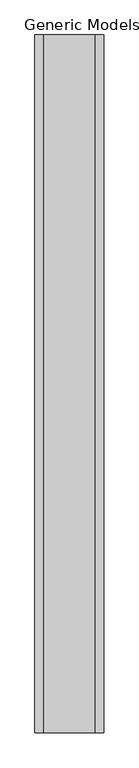
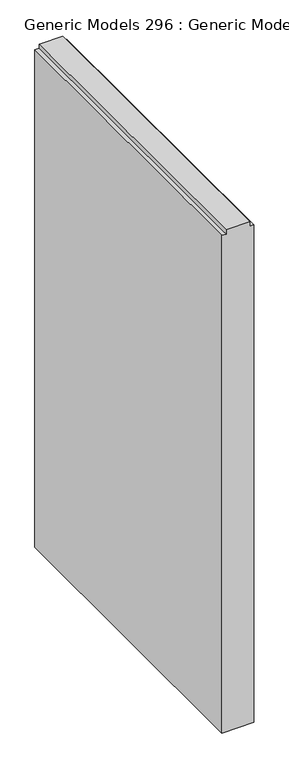
"""IFC4 building model written with IfcOpenShell, lengths in millimetres: proxy geometry, Generic Models 296 : Generic Models 208."""

from ifc_helpers import new_model, si_unit, frame, origin, place, context, project, spatial, polyline, outline, extrude, source, transform, mapped, element, save


def generic_models_296_generic_models_208_ffa1fc56(model_context):
    return source(origin(), model_context, "Body", "SweptSolid", [
        extrude(outline(polyline([(2082.8, 55034.6329676), (2099.865625, 55034.6329676), (2099.865625, 54945.7329676), (2082.8, 54945.7329676), (2082.8, 54929.8579676), (101.6, 54929.8579676), (101.6, 55050.5079676), (2082.8, 55050.5079676), (2082.8, 55034.6329676)])), frame((0.0, -228.7033818, 0.0), z_axis=(0.0, 1.0, 0.0), x_axis=(0.0, 0.0, 1.0)), (0.0, 0.0, 1.0), 1219.2),
    ])


if __name__ == "__main__":
    model = new_model("IFC4")
    model_context = context("Model", 3, world=origin())
    ifc_project = project(units=[si_unit("LENGTHUNIT", "METRE", prefix="MILLI")], contexts=[model_context])
    site = spatial("IfcSite", under=ifc_project)
    building = spatial("IfcBuilding", under=site)
    placement = place(None, origin())
    generic_models_296_generic_models_208_shape = generic_models_296_generic_models_208_ffa1fc56(model_context)
    element("IfcBuildingElementProxy", 1, Name="Generic Models 296 : Generic Models 208", ObjectType="Generic Models 296 : Generic Models 208", at=placement, inside=building, context=model_context, shape_type="MappedRepresentation", body=[
        mapped(generic_models_296_generic_models_208_shape, transform((0.0, 0.0, 0.0), x_axis=(1.0, 0.0, 0.0), y_axis=(0.0, 1.0, 0.0), z_axis=(0.0, 0.0, 1.0))),
    ])
    save(model, "model.ifc")

# Revit data of these elements
# Element 1 (IfcBuildingElementProxy, "Generic Models 296 : Generic Models 208")
#   Materials on its faces: "5/8\" GYP. BD"
# Materials
#   "5/8\" GYP. BD": class "Generic", colour RGB 171 170 168, transparency 0, Description = "Gypsum Wall Board", Cost = 0
